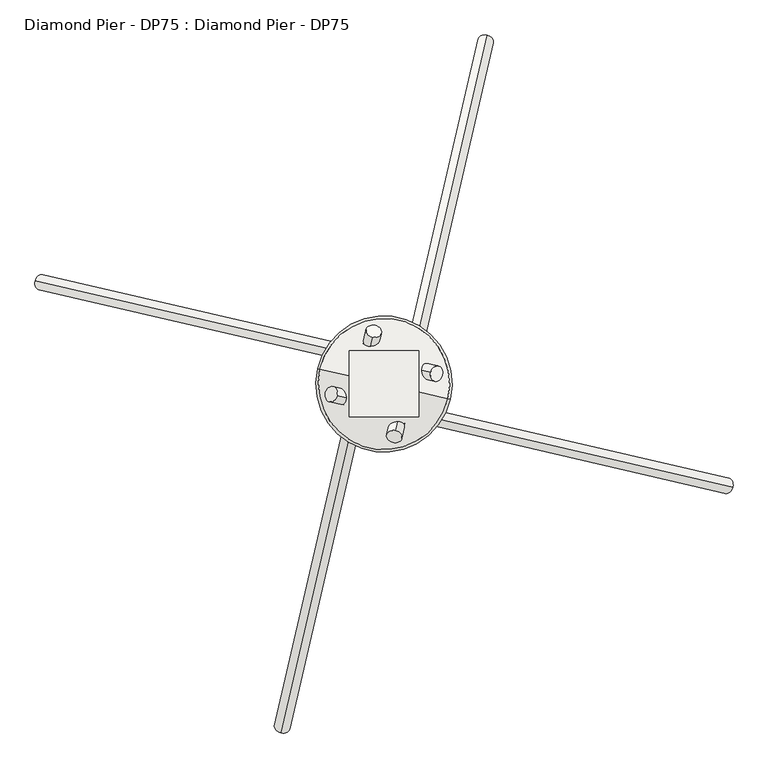
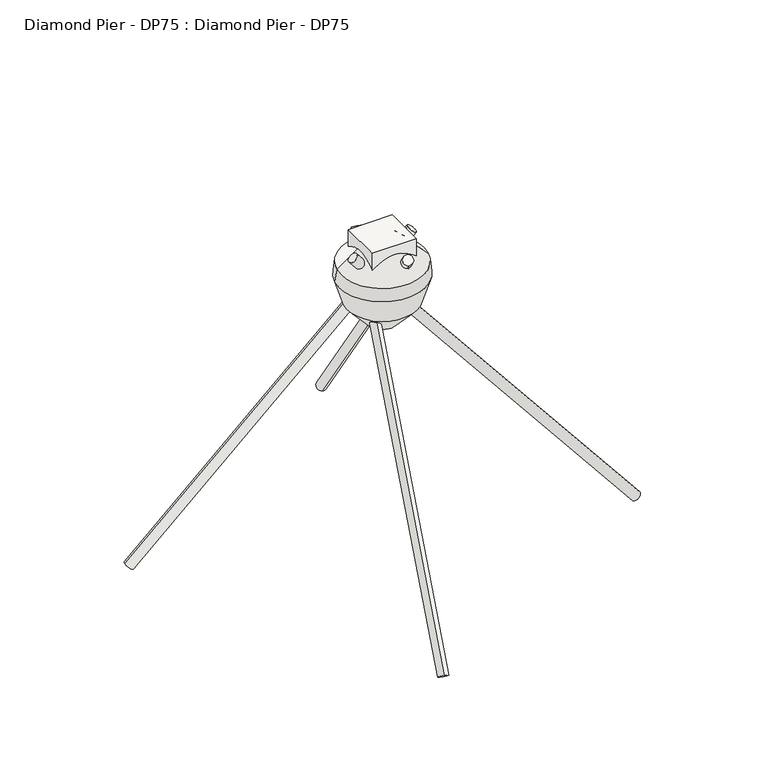
"""IFC4 building model written with IfcOpenShell, lengths in millimetres: slab geometry, Diamond Pier - DP75 : Diamond Pier - DP75."""

import ifcopenshell
import ifcopenshell.guid

model = None  # the IFC model being written
_history = None  # IfcOwnerHistory: only IFC2X3 demands one
_inside = {}  # id of a spatial element -> (the spatial element, [elements in it])
_under = {}  # id of a project, library or spatial element -> (it, [spatial elements below it])
_declared = {}  # id of a project -> (the project, [libraries it declares])
_typed = {}  # id of a type object -> (the type object, [elements of that type])
_made_of = {}  # id of a material, layer set ... -> (it, [elements and type objects made of it])


def new_model(schema):
    """Start an empty IFC model of exactly this schema.

    Asked for "IFC4X3", IfcOpenShell would pick the latest addendum, in which some entities
    have other attributes; the version numbers below select the first issue.
    IFC2X3 requires an IfcOwnerHistory on every rooted entity: one is made here for all.
    """
    global model, _history
    if schema == "IFC4X3":
        model = ifcopenshell.file(schema_version=(4, 3, 0, 0))
    else:
        model = ifcopenshell.file(schema=schema)
    _inside.clear()
    _under.clear()
    _declared.clear()
    _typed.clear()
    _made_of.clear()
    _history = None
    if model.schema == "IFC2X3":
        org = make("IfcOrganization", Name="unknown")
        user = make(
            "IfcPersonAndOrganization",
            ThePerson=make("IfcPerson", FamilyName="unknown"),
            TheOrganization=org,
        )
        app = make(
            "IfcApplication",
            ApplicationDeveloper=org,
            Version="unknown",
            ApplicationFullName="unknown",
            ApplicationIdentifier="unknown",
        )
        _history = make(
            "IfcOwnerHistory",
            OwningUser=user,
            OwningApplication=app,
            ChangeAction="ADDED",
            CreationDate=0,
        )
    return model


def make(cls, **values):
    """One entity of the class cls with the attributes given. An attribute that is None is left unset."""
    return model.create_entity(
        cls, **{name: value for name, value in values.items() if value is not None}
    )


def rooted(cls, **values):
    """An entity with a GlobalId (a new one), such as an element, a storey or a relation."""
    return make(cls, GlobalId=ifcopenshell.guid.new(), OwnerHistory=_history, **values)


def si_unit(unit_type, name, prefix=None):
    """IfcSIUnit, for example si_unit("LENGTHUNIT", "METRE", prefix="MILLI")."""
    return make("IfcSIUnit", UnitType=unit_type, Prefix=prefix, Name=name)


def assignment(units):
    """IfcUnitAssignment: the units of a project."""
    return None if units is None else make("IfcUnitAssignment", Units=units)


def point(xyz):
    """IfcCartesianPoint."""
    return None if xyz is None else make("IfcCartesianPoint", Coordinates=xyz)


def direction(xyz):
    """IfcDirection."""
    return None if xyz is None else make("IfcDirection", DirectionRatios=xyz)


def frame(location, z_axis=None, x_axis=None):
    """IfcAxis2Placement3D, a coordinate frame: its origin and axes. An axis left out is left unset."""
    return make(
        "IfcAxis2Placement3D",
        Location=point(location),
        Axis=direction(z_axis),
        RefDirection=direction(x_axis),
    )


def frame_2d(location, x_axis=None):
    """IfcAxis2Placement2D, a coordinate frame in the plane: its origin and x axis."""
    return make(
        "IfcAxis2Placement2D", Location=point(location), RefDirection=direction(x_axis)
    )


def origin():
    """The frame at (0, 0, 0) with its axes left unset."""
    return frame((0.0, 0.0, 0.0))


def place(relative_to, where):
    """IfcLocalPlacement: puts the frame where relative to a parent placement (None: the world)."""
    return make(
        "IfcLocalPlacement", PlacementRelTo=relative_to, RelativePlacement=where
    )


def context(
    kind, dimensions, precision=None, world=None, true_north=None, identifier=None
):
    """IfcGeometricRepresentationContext, for example the 3D "Model" context."""
    return make(
        "IfcGeometricRepresentationContext",
        ContextIdentifier=identifier,
        ContextType=kind,
        CoordinateSpaceDimension=dimensions,
        Precision=precision,
        WorldCoordinateSystem=world,
        TrueNorth=true_north,
    )


def project(units=None, contexts=None):
    """IfcProject with its units and contexts."""
    return rooted(
        "IfcProject",
        Name="project",
        RepresentationContexts=contexts,
        UnitsInContext=assignment(units),
    )


def spatial(cls, under=None, at=None, **own):
    """A site, building, storey or space (cls), placed at a placement, below another one or the project."""
    s = rooted(cls, ObjectPlacement=at, **own)
    if under is not None:
        _under.setdefault(under.id(), (under, []))[1].append(s)
    return s


def polyline(points):
    """IfcPolyline through the points."""
    return make("IfcPolyline", Points=[point(p) for p in points])


def circle_curve(where, radius):
    """IfcCircle in the frame where."""
    return make("IfcCircle", Position=where, Radius=radius)


def trimmed(basis, trim1, trim2, sense, master):
    """IfcTrimmedCurve: the piece of a basis curve between two trims."""
    return make(
        "IfcTrimmedCurve",
        BasisCurve=basis,
        Trim1=trim1,
        Trim2=trim2,
        SenseAgreement=sense,
        MasterRepresentation=master,
    )


def segment(curve, same_sense, transition):
    """IfcCompositeCurveSegment."""
    return make(
        "IfcCompositeCurveSegment",
        Transition=transition,
        SameSense=same_sense,
        ParentCurve=curve,
    )


def composite_curve(segments, self_intersect=None):
    """IfcCompositeCurve: segments joined end to end."""
    return make("IfcCompositeCurve", Segments=segments, SelfIntersect=self_intersect)


def outline(outer, holes=None, kind="AREA"):
    """IfcArbitraryClosedProfileDef: a profile drawn as a closed curve; with holes, ...WithVoids."""
    if holes is None:
        return make("IfcArbitraryClosedProfileDef", ProfileType=kind, OuterCurve=outer)
    return make(
        "IfcArbitraryProfileDefWithVoids",
        ProfileType=kind,
        OuterCurve=outer,
        InnerCurves=holes,
    )


def extrude(swept, where, along, depth):
    """IfcExtrudedAreaSolid: the profile swept, set in the frame where, extruded along a direction by depth."""
    return make(
        "IfcExtrudedAreaSolid",
        SweptArea=swept,
        Position=where,
        ExtrudedDirection=direction(along),
        Depth=depth,
    )


def shape(context_of_items, identifier, shape_type, items):
    """IfcShapeRepresentation: the items that make up one representation, for example the "Body"."""
    return make(
        "IfcShapeRepresentation",
        ContextOfItems=context_of_items,
        RepresentationIdentifier=identifier,
        RepresentationType=shape_type,
        Items=items,
    )


def source(mapping_origin, context_of_items, identifier, shape_type, items):
    """IfcRepresentationMap: a shape defined once, which mapped items show again and again."""
    return make(
        "IfcRepresentationMap",
        MappingOrigin=mapping_origin,
        MappedRepresentation=shape(context_of_items, identifier, shape_type, items),
    )


def transform(
    local_origin,
    x_axis=None,
    y_axis=None,
    z_axis=None,
    scale=None,
    scale2=None,
    scale3=None,
    uniform=True,
):
    """IfcCartesianTransformationOperator3D, or its non-uniform kind. x_axis, y_axis, z_axis: its Axis1, 2, 3."""
    if uniform:
        return make(
            "IfcCartesianTransformationOperator3D",
            Axis1=direction(x_axis),
            Axis2=direction(y_axis),
            LocalOrigin=point(local_origin),
            Scale=scale,
            Axis3=direction(z_axis),
        )
    return make(
        "IfcCartesianTransformationOperator3DnonUniform",
        Axis1=direction(x_axis),
        Axis2=direction(y_axis),
        LocalOrigin=point(local_origin),
        Scale=scale,
        Axis3=direction(z_axis),
        Scale2=scale2,
        Scale3=scale3,
    )


def mapped(mapping_source, mapping_target):
    """IfcMappedItem: shows the shape of a source again, moved by a transform."""
    return make(
        "IfcMappedItem", MappingSource=mapping_source, MappingTarget=mapping_target
    )


def made_of(thing, what):
    """Note that an element or type object is made of a material, layer set ...; save() writes the relation."""
    if what is not None:
        _made_of.setdefault(what.id(), (what, []))[1].append(thing)
    return thing


def element(
    cls,
    number,
    at=None,
    inside=None,
    cuts=None,
    type_object=None,
    material=None,
    context=None,
    identifier="Body",
    shape_type=None,
    held_by="IfcProductDefinitionShape",
    body=None,
    shapes=None,
    **own,
):
    """One element of the class cls, such as IfcWall. Its Tag is "e" and its number.

    at: its placement. inside: the storey or other place that contains it. cuts: it is an
    opening in that element (IfcRelVoidsElement). A single representation is given by context,
    identifier, shape_type and body (its items); several are given by shapes. held_by: the class
    of the entity that holds the representations. save() writes the other relations.
    """
    e = rooted(cls, Tag="e%d" % number, ObjectPlacement=at, **own)
    if body is not None:
        shapes = [shape(context, identifier, shape_type, body)]
    if shapes is not None:
        e.Representation = make(held_by, Representations=shapes)
    if inside is not None:
        _inside.setdefault(inside.id(), (inside, []))[1].append(e)
    if cuts is not None:
        rooted(
            "IfcRelVoidsElement", RelatingBuildingElement=cuts, RelatedOpeningElement=e
        )
    if type_object is not None:
        _typed.setdefault(type_object.id(), (type_object, []))[1].append(e)
    return made_of(e, material)


def aggregate(whole, parts):
    """IfcRelAggregates: a whole, such as a stair, and the parts it consists of."""
    return rooted("IfcRelAggregates", RelatingObject=whole, RelatedObjects=parts)


def save(model, path):
    """Write the relations noted so far, then the file.

    IfcRelAggregates (storeys below a building ...), IfcRelContainedInSpatialStructure (elements
    in a storey), IfcRelDefinesByType, IfcRelAssociatesMaterial and IfcRelDeclares: one each for
    every whole, place, type object, material and project.
    """
    for whole, parts in _under.values():
        aggregate(whole, parts)
    for where, things in _inside.values():
        rooted(
            "IfcRelContainedInSpatialStructure",
            RelatedElements=things,
            RelatingStructure=where,
        )
    for kind, things in _typed.values():
        rooted("IfcRelDefinesByType", RelatedObjects=things, RelatingType=kind)
    for what, things in _made_of.values():
        rooted("IfcRelAssociatesMaterial", RelatedObjects=things, RelatingMaterial=what)
    for by, libraries in _declared.values():
        rooted("IfcRelDeclares", RelatingContext=by, RelatedDefinitions=libraries)
    model.write(path)


def plane_surface(at):
    """IfcPlane: the flat surface through the origin of the frame at, square to its z axis."""
    return make("IfcPlane", Position=at)


def revolved_surface(curve, axis_point, axis_direction):
    """IfcSurfaceOfRevolution: the curve turned about the line through axis_point along axis_direction."""
    return make(
        "IfcSurfaceOfRevolution",
        SweptCurve=make("IfcArbitraryOpenProfileDef", ProfileType="CURVE", Curve=curve),
        AxisPosition=make("IfcAxis1Placement", Location=point(axis_point), Axis=direction(axis_direction)),
    )


def advanced_brep(points, edges, surfaces, faces):
    """IfcAdvancedBrep: a solid bounded by faces that lie on surfaces and meet in shared edges.

    An edge is (start, end): straight between two places in points (the first is 0);
    or (start, end, curve); or (start, end, curve, False) where it runs against its curve.
    A face is (place in surfaces, loops), or (place, loops, False) where it looks against
    its surface's normal. A loop lists edges by number (the first is 1), with a minus sign
    where the edge is run from its end to its start. The first loop is the outer one.
    """
    corners = [point(p) for p in points]
    vertices = [make("IfcVertexPoint", VertexGeometry=c) for c in corners]
    made = []
    for start, end, *more in edges:
        made.append(
            make(
                "IfcEdgeCurve",
                EdgeStart=vertices[start],
                EdgeEnd=vertices[end],
                EdgeGeometry=more[0] if more else make("IfcPolyline", Points=[corners[start], corners[end]]),
                SameSense=more[1] if len(more) > 1 else True,
            )
        )
    hull = []
    for where, loops, *sense in faces:
        bounds = []
        for j, loop in enumerate(loops):
            ring = [make("IfcOrientedEdge", EdgeElement=made[abs(k) - 1], Orientation=k > 0) for k in loop]
            bounds.append(
                make(
                    "IfcFaceOuterBound" if j == 0 else "IfcFaceBound",
                    Bound=make("IfcEdgeLoop", EdgeList=ring),
                    Orientation=True,
                )
            )
        hull.append(make("IfcAdvancedFace", Bounds=bounds, FaceSurface=surfaces[where], SameSense=sense[0] if sense else True))
    return make("IfcAdvancedBrep", Outer=make("IfcClosedShell", CfsFaces=hull))


def diamond_pier_dp75_diamond_pier_dp75_ae65de88(model_context):
    return source(origin(), model_context, "Body", "SolidModel", [
        extrude(outline(composite_curve([segment(trimmed(circle_curve(frame_2d((1e-07, -15.875)), 15.875), [point((1e-07, -31.7500001))], [point((0.0, 0.0))], False, "CARTESIAN"), True, "CONTINUOUS"), segment(trimmed(circle_curve(frame_2d((1e-07, -15.875)), 15.875), [point((0.0, 0.0))], [point((1e-07, -31.7500001))], False, "CARTESIAN"), True, "CONTINUOUS")], self_intersect=False)), frame((-207.7929333, -703.2724242, -991.3584593), z_axis=(0.14520854647133766, 0.628002114484006, 0.7645441924671841), x_axis=(-0.9742942350214497, 0.2252792569322976, 0.0)), (0.0, 0.0, 1.0), 1270.0),
        extrude(outline(composite_curve([segment(trimmed(circle_curve(frame_2d((1e-07, -15.875)), 15.875), [point((1e-07, -31.7500001))], [point((0.0, 0.0))], False, "CARTESIAN"), True, "CONTINUOUS"), segment(trimmed(circle_curve(frame_2d((1e-07, -15.875)), 15.875), [point((0.0, 0.0))], [point((1e-07, -31.7500001))], False, "CARTESIAN"), True, "CONTINUOUS")], self_intersect=False)), frame((-703.2724242, 207.7929333, -991.3584593), z_axis=(0.6280021144840067, -0.14520854647133485, 0.7645441924671843), x_axis=(0.22527925693229323, 0.9742942350214507, 0.0)), (0.0, 0.0, 1.0), 1270.0),
        extrude(outline(composite_curve([segment(trimmed(circle_curve(frame_2d((1e-07, -15.875)), 15.875), [point((1e-07, -31.7500001))], [point((0.0, 0.0))], False, "CARTESIAN"), True, "CONTINUOUS"), segment(trimmed(circle_curve(frame_2d((1e-07, -15.875)), 15.875), [point((0.0, 0.0))], [point((1e-07, -31.7500001))], False, "CARTESIAN"), True, "CONTINUOUS")], self_intersect=False)), frame((207.7929333, 703.2724242, -991.3584593), z_axis=(-0.14520854647133596, -0.6280021144840063, 0.7645441924671844), x_axis=(0.9742942350214504, -0.22527925693229495, 0.0)), (0.0, 0.0, 1.0), 1270.0),
        extrude(outline(composite_curve([segment(trimmed(circle_curve(frame_2d((1e-07, -15.875)), 15.875), [point((1e-07, -31.7500001))], [point((0.0, 0.0))], False, "CARTESIAN"), True, "CONTINUOUS"), segment(trimmed(circle_curve(frame_2d((1e-07, -15.875)), 15.875), [point((0.0, 0.0))], [point((1e-07, -31.7500001))], False, "CARTESIAN"), True, "CONTINUOUS")], self_intersect=False)), frame((703.2724242, -207.7929333, -991.3584593), z_axis=(-0.6280021144840057, 0.14520854647133877, 0.7645441924671843), x_axis=(-0.22527925693229922, -0.9742942350214493, 0.0)), (0.0, 0.0, 1.0), 1270.0),
        advanced_brep(
        [(-108.3324504, 25.0489565, -217.3055075), (108.3324504, -25.0489565, -217.3055075), (42.5837569, -9.8463449, -291.7305661), (-42.5837569, 9.8463449, -291.7305661), (-133.8544614, 30.950233, -132.1736467), (133.8544614, -30.950233, -132.1736467), (-128.9734508, 29.821631, -90.9283538), (128.9734508, -29.821631, -90.9283538), (-48.2749795, 11.1622866, -12.7), (48.2749795, -11.1622866, -12.7), (0.0, 0.0, -12.7), (0.0, 0.0, -292.024192)],
        [
            (0, 1, circle_curve(frame((0.0, 0.0, -217.3055075), z_axis=(0.0, 0.0, -1.0), x_axis=(0.9742942350214493, -0.22527925693229933, 0.0)), 111.1906922)),
            (1, 2),
            (2, 3, circle_curve(frame((0.0, 0.0, -291.7305661), z_axis=(0.0, 0.0, 1.0), x_axis=(0.9742942350214493, -0.22527925693229933, 0.0)), 43.7072861)),
            (3, 0),
            (1, 0, circle_curve(frame((0.0, 0.0, -217.3055075), z_axis=(0.0, 0.0, -1.0), x_axis=(0.9742942350214493, -0.22527925693229933, 0.0)), 111.1906922)),
            (3, 2, circle_curve(frame((0.0, 0.0, -291.7305661), z_axis=(0.0, 0.0, 1.0), x_axis=(0.9742942350214493, -0.22527925693229933, 0.0)), 43.7072861)),
            (4, 5, circle_curve(frame((0.0, 0.0, -132.1736467), z_axis=(0.0, 0.0, -1.0), x_axis=(0.9742942350214493, -0.22527925693229933, 0.0)), 137.3860755)),
            (5, 1),
            (0, 4),
            (5, 4, circle_curve(frame((0.0, 0.0, -132.1736467), z_axis=(0.0, 0.0, -1.0), x_axis=(0.9742942350214493, -0.22527925693229933, 0.0)), 137.3860755)),
            (6, 7, circle_curve(frame((0.0, 0.0, -90.9283538), z_axis=(0.0, 0.0, -1.0), x_axis=(0.9742942350214493, -0.22527925693229933, 0.0)), 132.3762845)),
            (7, 5),
            (4, 6),
            (7, 6, circle_curve(frame((0.0, 0.0, -90.9283538), z_axis=(0.0, 0.0, -1.0), x_axis=(0.9742942350214493, -0.22527925693229933, 0.0)), 132.3762845)),
            (8, 9, circle_curve(frame((0.0, 0.0, -12.7), z_axis=(0.0, 0.0, -1.0), x_axis=(0.9742942350214493, -0.22527925693229933, 0.0)), 49.5486659)),
            (9, 7),
            (6, 8),
            (9, 8, circle_curve(frame((0.0, 0.0, -12.7), z_axis=(0.0, 0.0, -1.0), x_axis=(0.9742942350214493, -0.22527925693229933, 0.0)), 49.5486659)),
            (10, 9),
            (8, 10),
            (2, 11),
            (11, 3),
        ],
        [
            revolved_surface(polyline([(42.5837569, -9.8463449, -291.7305661), (108.3324504, -25.0489565, -217.3055075)]), (0.0, 0.0, -12.7), (0.0, 0.0, 1.0)),
            revolved_surface(polyline([(108.3324504, -25.0489565, -217.3055075), (133.8544614, -30.950233, -132.1736467)]), (0.0, 0.0, -12.7), (0.0, 0.0, 1.0)),
            revolved_surface(polyline([(133.8544614, -30.950233, -132.1736467), (128.9734508, -29.821631, -90.9283538)]), (0.0, 0.0, -12.7), (0.0, 0.0, 1.0)),
            revolved_surface(polyline([(128.9734508, -29.821631, -90.9283538), (48.2749795, -11.1622866, -12.7)]), (0.0, 0.0, -12.7), (0.0, 0.0, 1.0)),
            plane_surface(frame((0.0, 0.0, -12.7), z_axis=(0.0, 0.0, 1.0), x_axis=(0.9742942350214493, -0.22527925693229933, 0.0))),
            revolved_surface(polyline([(0.0, 0.0, -292.024192), (42.5837569, -9.8463449, -291.7305661)]), (0.0, 0.0, -12.7), (0.0, 0.0, 1.0)),
        ],
        [
            (0, [[1, 2, 3, 4]]),
            (0, [[5, -4, 6, -2]]),
            (1, [[7, 8, -1, 9]]),
            (1, [[10, -9, -5, -8]]),
            (2, [[11, 12, -7, 13]]),
            (2, [[14, -13, -10, -12]]),
            (3, [[15, 16, -11, 17]]),
            (3, [[18, -17, -14, -16]]),
            (4, [[19, -15, 20]]),
            (4, [[-20, -18, -19]]),
            (5, [[-3, 21, 22]]),
            (5, [[-6, -22, -21]]),
        ],
    ),
        extrude(outline(polyline([(70.369164, 66.5326915), (70.369164, -66.5326915), (-70.369164, -66.5326915), (-70.369164, 66.5326915), (70.369164, 66.5326915)])), frame((0.0, 0.0, -87.3372243), z_axis=(0.0, 0.0, 1.0), x_axis=(1.0, 0.0, 0.0)), (0.0, 0.0, 1.0), 87.3372243),
    ])


if __name__ == "__main__":
    model = new_model("IFC4")
    model_context = context("Model", 3, world=origin())
    ifc_project = project(units=[si_unit("LENGTHUNIT", "METRE", prefix="MILLI")], contexts=[model_context])
    site = spatial("IfcSite", under=ifc_project)
    building = spatial("IfcBuilding", under=site)
    placement = place(None, origin())
    diamond_pier_dp75_diamond_pier_dp75_shape = diamond_pier_dp75_diamond_pier_dp75_ae65de88(model_context)
    element("IfcSlab", 1, ObjectType="Diamond Pier - DP75 : Diamond Pier - DP75", at=placement, inside=building, context=model_context, shape_type="MappedRepresentation", body=[
        mapped(diamond_pier_dp75_diamond_pier_dp75_shape, transform((0.0, 0.0, 0.0), x_axis=(1.0, 0.0, 0.0), y_axis=(0.0, 1.0, 0.0), z_axis=(0.0, 0.0, 1.0))),
    ])
    save(model, "model.ifc")

# Revit data of these elements
# Type "Diamond Pier - DP75 : Diamond Pier - DP75"
#   Assembly Code = "A1010100"
#   Structural Material = DIAMOND PIER DP-50/50 - (3300# B.L.C. AT 1500PSF SOILS, 4400# B.L.C. AT 2000PSF SOILS)
# Element 1 (IfcSlab, "Diamond Pier - DP75 : Diamond Pier - DP75")
#   Materials on its faces: "DIAMOND PIER DP-50/50 - (3300# B.L.C. AT 1500PSF SOILS, 4400# B.L.C. AT 2000PSF SOILS)"
# Materials
#   "DIAMOND PIER DP-50/50 - (3300# B.L.C. AT 1500PSF SOILS, 4400# B.L.C. AT 2000PSF SOILS)": class "Generic", colour RGB 195 195 195, transparency 0, Cost = 0
